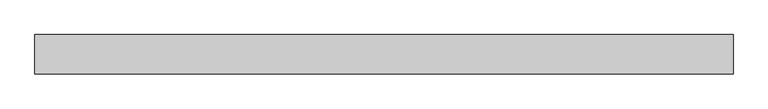
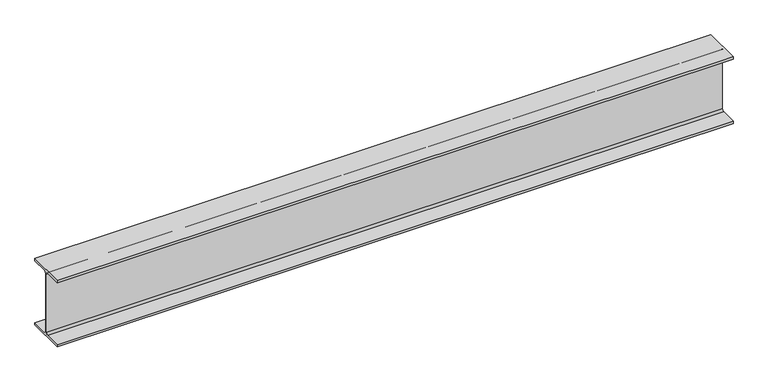
"""IFC4 building model written with IfcOpenShell, lengths in millimetres: beam geometry, Old_Steel Beam_H-KSD3502 : H_SB_ASB_H-250×125x6x9."""

from ifc_helpers import new_model, si_unit, point, frame, frame_2d, origin, place, context, project, spatial, polyline, circle_curve, trimmed, segment, composite_curve, outline, extrude, source, transform, mapped, element, save


def beam_6a67d305(model_context):
    return source(origin(), model_context, "Body", "SweptSolid", [
        extrude(outline(composite_curve([segment(polyline([(82.5, -141.5), (82.5, -151.7), (-82.5, -151.7), (-82.5, -141.5), (-11.9, -141.5)]), True, "CONTINUOUS"), segment(trimmed(circle_curve(frame_2d((-11.9, -132.6)), 8.9), [point((-11.9, -141.5))], [point((-3.0, -132.6))], True, "CARTESIAN"), True, "CONTINUOUS"), segment(polyline([(-3.0, -132.6), (-3.0, 132.6)]), True, "CONTINUOUS"), segment(trimmed(circle_curve(frame_2d((-11.9, 132.6)), 8.9), [point((-3.0, 132.6))], [point((-11.9, 141.5))], True, "CARTESIAN"), True, "CONTINUOUS"), segment(polyline([(-11.9, 141.5), (-82.5, 141.5), (-82.5, 151.7), (82.5, 151.7), (82.5, 141.5), (11.9, 141.5)]), True, "CONTINUOUS"), segment(trimmed(circle_curve(frame_2d((11.9, 132.6)), 8.9), [point((11.9, 141.5))], [point((3.0, 132.6))], True, "CARTESIAN"), True, "CONTINUOUS"), segment(polyline([(3.0, 132.6), (3.0, -132.6)]), True, "CONTINUOUS"), segment(trimmed(circle_curve(frame_2d((11.9, -132.6)), 8.9), [point((3.0, -132.6))], [point((11.9, -141.5))], True, "CARTESIAN"), True, "CONTINUOUS"), segment(polyline([(11.9, -141.5), (82.5, -141.5)]), True, "CONTINUOUS")], self_intersect=False)), frame((-1529.8000466, 0.0, 0.0), z_axis=(1.0, 0.0, 0.0), x_axis=(0.0, 1.0, 0.0)), (0.0, 0.0, 1.0), 2912.0982036),
    ])


if __name__ == "__main__":
    model = new_model("IFC4")
    model_context = context("Model", 3, world=origin())
    ifc_project = project(units=[si_unit("LENGTHUNIT", "METRE", prefix="MILLI")], contexts=[model_context])
    site = spatial("IfcSite", under=ifc_project)
    building = spatial("IfcBuilding", under=site)
    placement = place(None, origin())
    beam_shape = beam_6a67d305(model_context)
    element("IfcBeam", 1, ObjectType="Old_Steel Beam_H-KSD3502 : H_SB_ASB_H-250×125x6x9", at=placement, inside=building, context=model_context, shape_type="MappedRepresentation", body=[
        mapped(beam_shape, transform((0.0, 0.0, 0.0), x_axis=(1.0, 0.0, 0.0), y_axis=(0.0, 1.0, 0.0), z_axis=(0.0, 0.0, 1.0))),
    ])
    save(model, "model.ifc")

# Revit data of these elements
# Type "Old_Steel Beam_H-KSD3502 : H_SB_ASB_H-250×125x6x9"
#   Width = 12.5 cm
#   Web Thickness = 0.6 cm
#   Web Fillet = 1.2 cm
#   Warping Constant = 42539.8 cm⁶
#   Torsional Moment of Inertia = 7.8102 cm⁴
#   Torsional Modulus = 1.0 cm³
#   Section Area = 37.66 cm²
#   Plastic Modulus weak axis = 73.1 cm³
#   Plastic Modulus strong axis = 366.0 cm³
#   Perimeter = 0.97 m²/m
#   Nominal Weight = 29.60 kgf/m
#   Moment of Inertia weak axis = 294.00 cm⁴
#   Moment of Inertia strong axis = 4050.00 cm⁴
#   Height = 25.0 cm
#   Flange Thickness = 0.9 cm
#   Elastic Modulus weak axis = 47.0 cm³
#   Elastic Modulus strong axis = 324.0 cm³
#   Centroid Vertical = 12.5 cm
#   Centroid Horizontal = 6.25 cm
#   Length [instance default] = 1.5240 m
#   Structural Material [instance default] = Steel, 45-345
#   Assembly Code = ""
# Element 1 (IfcBeam, "Old_Steel Beam_H-KSD3502 : H_SB_ASB_H-250×125x6x9")
#   Structural Material = none
# Materials
#   "Steel, 45-345": class "Metal", colour RGB 189 187 185, transparency 0, Description = "Steel 345 MPa", Cost = 0
